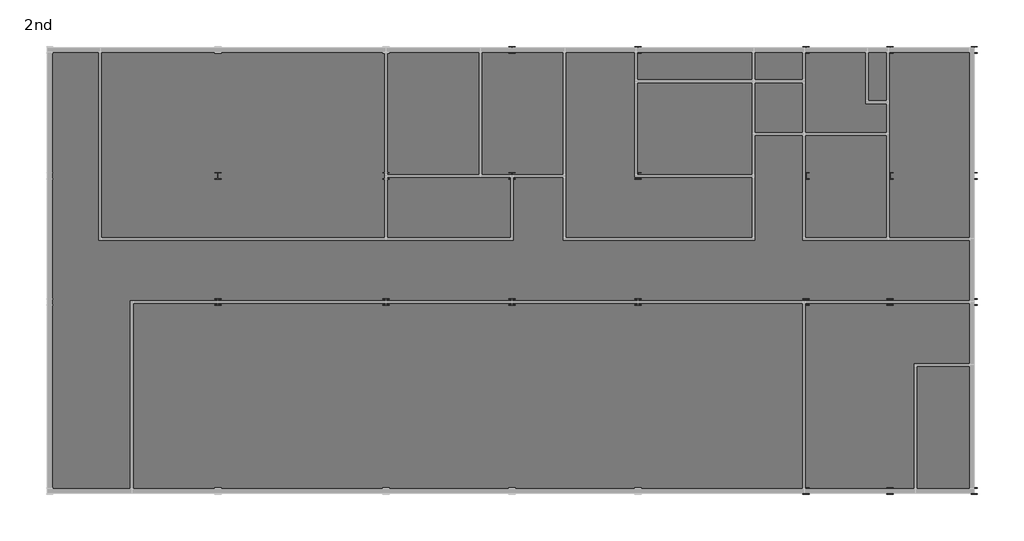
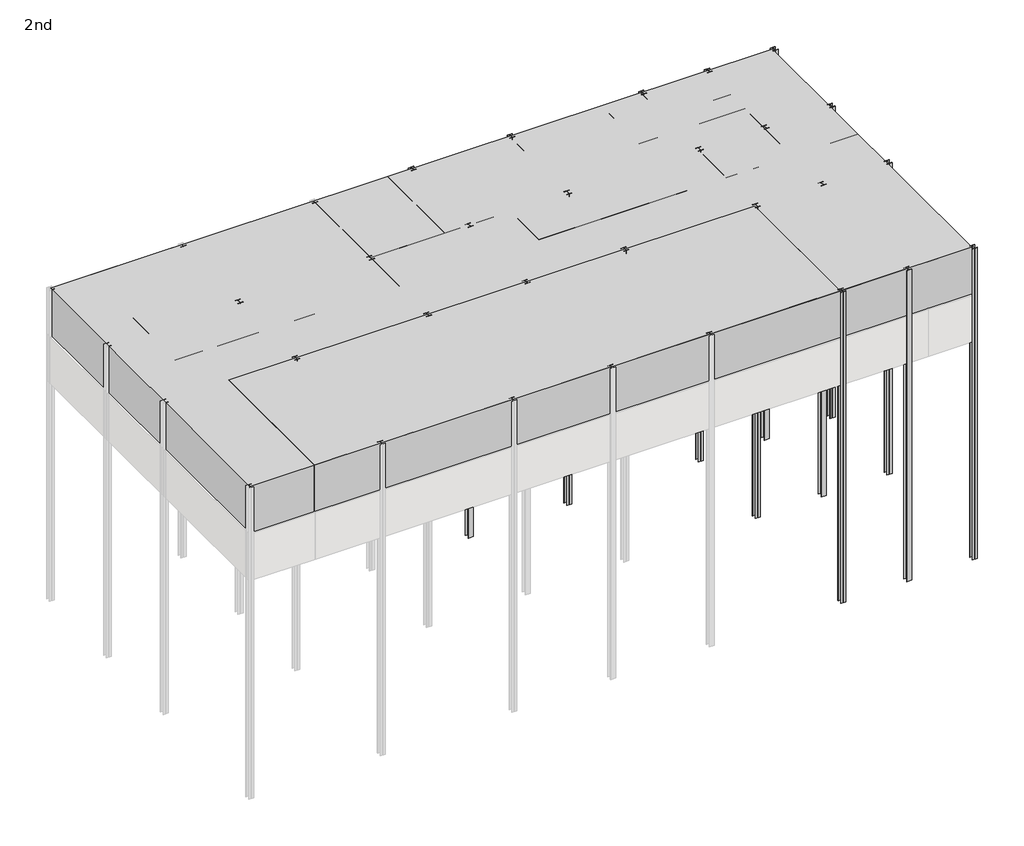
# One storey, part 3 of 3: 17 proxies, 16 columns.
"""IFC4 building model written with IfcOpenShell, lengths in millimetres."""

import ifcopenshell
import ifcopenshell.guid

model = None  # the IFC model being written
_history = None  # IfcOwnerHistory: only IFC2X3 demands one
_inside = {}  # id of a spatial element -> (the spatial element, [elements in it])
_under = {}  # id of a project, library or spatial element -> (it, [spatial elements below it])
_declared = {}  # id of a project -> (the project, [libraries it declares])
_typed = {}  # id of a type object -> (the type object, [elements of that type])
_made_of = {}  # id of a material, layer set ... -> (it, [elements and type objects made of it])


def new_model(schema):
    """Start an empty IFC model of exactly this schema.

    Asked for "IFC4X3", IfcOpenShell would pick the latest addendum, in which some entities
    have other attributes; the version numbers below select the first issue.
    IFC2X3 requires an IfcOwnerHistory on every rooted entity: one is made here for all.
    """
    global model, _history
    if schema == "IFC4X3":
        model = ifcopenshell.file(schema_version=(4, 3, 0, 0))
    else:
        model = ifcopenshell.file(schema=schema)
    _inside.clear()
    _under.clear()
    _declared.clear()
    _typed.clear()
    _made_of.clear()
    _history = None
    if model.schema == "IFC2X3":
        org = make("IfcOrganization", Name="unknown")
        user = make(
            "IfcPersonAndOrganization",
            ThePerson=make("IfcPerson", FamilyName="unknown"),
            TheOrganization=org,
        )
        app = make(
            "IfcApplication",
            ApplicationDeveloper=org,
            Version="unknown",
            ApplicationFullName="unknown",
            ApplicationIdentifier="unknown",
        )
        _history = make(
            "IfcOwnerHistory",
            OwningUser=user,
            OwningApplication=app,
            ChangeAction="ADDED",
            CreationDate=0,
        )
    return model


def make(cls, **values):
    """One entity of the class cls with the attributes given. An attribute that is None is left unset."""
    return model.create_entity(
        cls, **{name: value for name, value in values.items() if value is not None}
    )


def rooted(cls, **values):
    """An entity with a GlobalId (a new one), such as an element, a storey or a relation."""
    return make(cls, GlobalId=ifcopenshell.guid.new(), OwnerHistory=_history, **values)


def si_unit(unit_type, name, prefix=None):
    """IfcSIUnit, for example si_unit("LENGTHUNIT", "METRE", prefix="MILLI")."""
    return make("IfcSIUnit", UnitType=unit_type, Prefix=prefix, Name=name)


def assignment(units):
    """IfcUnitAssignment: the units of a project."""
    return None if units is None else make("IfcUnitAssignment", Units=units)


def point(xyz):
    """IfcCartesianPoint."""
    return None if xyz is None else make("IfcCartesianPoint", Coordinates=xyz)


def direction(xyz):
    """IfcDirection."""
    return None if xyz is None else make("IfcDirection", DirectionRatios=xyz)


def frame(location, z_axis=None, x_axis=None):
    """IfcAxis2Placement3D, a coordinate frame: its origin and axes. An axis left out is left unset."""
    return make(
        "IfcAxis2Placement3D",
        Location=point(location),
        Axis=direction(z_axis),
        RefDirection=direction(x_axis),
    )


def frame_2d(location, x_axis=None):
    """IfcAxis2Placement2D, a coordinate frame in the plane: its origin and x axis."""
    return make(
        "IfcAxis2Placement2D", Location=point(location), RefDirection=direction(x_axis)
    )


def origin():
    """The frame at (0, 0, 0) with its axes left unset."""
    return frame((0.0, 0.0, 0.0))


def origin_with_axes():
    """The frame at (0, 0, 0) with the z axis (0, 0, 1) and the x axis (1, 0, 0) written out."""
    return frame((0.0, 0.0, 0.0), z_axis=(0.0, 0.0, 1.0), x_axis=(1.0, 0.0, 0.0))


def place(relative_to, where):
    """IfcLocalPlacement: puts the frame where relative to a parent placement (None: the world)."""
    return make(
        "IfcLocalPlacement", PlacementRelTo=relative_to, RelativePlacement=where
    )


def context(
    kind, dimensions, precision=None, world=None, true_north=None, identifier=None
):
    """IfcGeometricRepresentationContext, for example the 3D "Model" context."""
    return make(
        "IfcGeometricRepresentationContext",
        ContextIdentifier=identifier,
        ContextType=kind,
        CoordinateSpaceDimension=dimensions,
        Precision=precision,
        WorldCoordinateSystem=world,
        TrueNorth=true_north,
    )


def project(units=None, contexts=None):
    """IfcProject with its units and contexts."""
    return rooted(
        "IfcProject",
        Name="project",
        RepresentationContexts=contexts,
        UnitsInContext=assignment(units),
    )


def spatial(cls, under=None, at=None, **own):
    """A site, building, storey or space (cls), placed at a placement, below another one or the project."""
    s = rooted(cls, ObjectPlacement=at, **own)
    if under is not None:
        _under.setdefault(under.id(), (under, []))[1].append(s)
    return s


def polyline(points):
    """IfcPolyline through the points."""
    return make("IfcPolyline", Points=[point(p) for p in points])


def circle_curve(where, radius):
    """IfcCircle in the frame where."""
    return make("IfcCircle", Position=where, Radius=radius)


def trimmed(basis, trim1, trim2, sense, master):
    """IfcTrimmedCurve: the piece of a basis curve between two trims."""
    return make(
        "IfcTrimmedCurve",
        BasisCurve=basis,
        Trim1=trim1,
        Trim2=trim2,
        SenseAgreement=sense,
        MasterRepresentation=master,
    )


def segment(curve, same_sense, transition):
    """IfcCompositeCurveSegment."""
    return make(
        "IfcCompositeCurveSegment",
        Transition=transition,
        SameSense=same_sense,
        ParentCurve=curve,
    )


def composite_curve(segments, self_intersect=None):
    """IfcCompositeCurve: segments joined end to end."""
    return make("IfcCompositeCurve", Segments=segments, SelfIntersect=self_intersect)


def outline(outer, holes=None, kind="AREA"):
    """IfcArbitraryClosedProfileDef: a profile drawn as a closed curve; with holes, ...WithVoids."""
    if holes is None:
        return make("IfcArbitraryClosedProfileDef", ProfileType=kind, OuterCurve=outer)
    return make(
        "IfcArbitraryProfileDefWithVoids",
        ProfileType=kind,
        OuterCurve=outer,
        InnerCurves=holes,
    )


def extrude(swept, where, along, depth):
    """IfcExtrudedAreaSolid: the profile swept, set in the frame where, extruded along a direction by depth."""
    return make(
        "IfcExtrudedAreaSolid",
        SweptArea=swept,
        Position=where,
        ExtrudedDirection=direction(along),
        Depth=depth,
    )


def shape(context_of_items, identifier, shape_type, items):
    """IfcShapeRepresentation: the items that make up one representation, for example the "Body"."""
    return make(
        "IfcShapeRepresentation",
        ContextOfItems=context_of_items,
        RepresentationIdentifier=identifier,
        RepresentationType=shape_type,
        Items=items,
    )


def source(mapping_origin, context_of_items, identifier, shape_type, items):
    """IfcRepresentationMap: a shape defined once, which mapped items show again and again."""
    return make(
        "IfcRepresentationMap",
        MappingOrigin=mapping_origin,
        MappedRepresentation=shape(context_of_items, identifier, shape_type, items),
    )


def transform(
    local_origin,
    x_axis=None,
    y_axis=None,
    z_axis=None,
    scale=None,
    scale2=None,
    scale3=None,
    uniform=True,
):
    """IfcCartesianTransformationOperator3D, or its non-uniform kind. x_axis, y_axis, z_axis: its Axis1, 2, 3."""
    if uniform:
        return make(
            "IfcCartesianTransformationOperator3D",
            Axis1=direction(x_axis),
            Axis2=direction(y_axis),
            LocalOrigin=point(local_origin),
            Scale=scale,
            Axis3=direction(z_axis),
        )
    return make(
        "IfcCartesianTransformationOperator3DnonUniform",
        Axis1=direction(x_axis),
        Axis2=direction(y_axis),
        LocalOrigin=point(local_origin),
        Scale=scale,
        Axis3=direction(z_axis),
        Scale2=scale2,
        Scale3=scale3,
    )


def mapped(mapping_source, mapping_target):
    """IfcMappedItem: shows the shape of a source again, moved by a transform."""
    return make(
        "IfcMappedItem", MappingSource=mapping_source, MappingTarget=mapping_target
    )


def made_of(thing, what):
    """Note that an element or type object is made of a material, layer set ...; save() writes the relation."""
    if what is not None:
        _made_of.setdefault(what.id(), (what, []))[1].append(thing)
    return thing


def element(
    cls,
    number,
    at=None,
    inside=None,
    cuts=None,
    type_object=None,
    material=None,
    context=None,
    identifier="Body",
    shape_type=None,
    held_by="IfcProductDefinitionShape",
    body=None,
    shapes=None,
    **own,
):
    """One element of the class cls, such as IfcWall. Its Tag is "e" and its number.

    at: its placement. inside: the storey or other place that contains it. cuts: it is an
    opening in that element (IfcRelVoidsElement). A single representation is given by context,
    identifier, shape_type and body (its items); several are given by shapes. held_by: the class
    of the entity that holds the representations. save() writes the other relations.
    """
    e = rooted(cls, Tag="e%d" % number, ObjectPlacement=at, **own)
    if body is not None:
        shapes = [shape(context, identifier, shape_type, body)]
    if shapes is not None:
        e.Representation = make(held_by, Representations=shapes)
    if inside is not None:
        _inside.setdefault(inside.id(), (inside, []))[1].append(e)
    if cuts is not None:
        rooted(
            "IfcRelVoidsElement", RelatingBuildingElement=cuts, RelatedOpeningElement=e
        )
    if type_object is not None:
        _typed.setdefault(type_object.id(), (type_object, []))[1].append(e)
    return made_of(e, material)


def aggregate(whole, parts):
    """IfcRelAggregates: a whole, such as a stair, and the parts it consists of."""
    return rooted("IfcRelAggregates", RelatingObject=whole, RelatedObjects=parts)


def save(model, path):
    """Write the relations noted so far, then the file.

    IfcRelAggregates (storeys below a building ...), IfcRelContainedInSpatialStructure (elements
    in a storey), IfcRelDefinesByType, IfcRelAssociatesMaterial and IfcRelDeclares: one each for
    every whole, place, type object, material and project.
    """
    for whole, parts in _under.values():
        aggregate(whole, parts)
    for where, things in _inside.values():
        rooted(
            "IfcRelContainedInSpatialStructure",
            RelatedElements=things,
            RelatingStructure=where,
        )
    for kind, things in _typed.values():
        rooted("IfcRelDefinesByType", RelatedObjects=things, RelatingType=kind)
    for what, things in _made_of.values():
        rooted("IfcRelAssociatesMaterial", RelatedObjects=things, RelatingMaterial=what)
    for by, libraries in _declared.values():
        rooted("IfcRelDeclares", RelatingContext=by, RelatedDefinitions=libraries)
    model.write(path)


def generic_models_29bcd6f9(model_context):
    return source(origin(), model_context, "Body", "SweptSolid", [
        extrude(outline(polyline([(2000.0, 4500.0), (2000.0, -4500.0), (-2000.0, -4500.0), (-2000.0, 4500.0), (2000.0, 4500.0)])), origin_with_axes(), (0.0, 0.0, 1.0), 6000.0),
    ])


def generic_models_5634f436(model_context):
    return source(origin(), model_context, "Body", "SweptSolid", [
        extrude(outline(polyline([(1350.0, 3000.0), (1350.0, -3000.0), (-1350.0, -3000.0), (-1350.0, 3000.0), (1350.0, 3000.0)])), origin_with_axes(), (0.0, 0.0, 1.0), 6000.0),
    ])


def generic_models_71e2440f(model_context):
    return source(origin(), model_context, "Body", "SweptSolid", [
        extrude(outline(polyline([(500.0, 1250.0), (500.0, -1250.0), (-500.0, -1250.0), (-500.0, 1250.0), (500.0, 1250.0)])), origin_with_axes(), (0.0, 0.0, 1.0), 6000.0),
    ])


def generic_models_57c7875f(model_context):
    return source(origin(), model_context, "Body", "SweptSolid", [
        extrude(outline(polyline([(4500.0, 16000.0), (4500.0, -16000.0), (-4500.0, -16000.0), (-4500.0, 16000.0), (4500.0, 16000.0)])), origin_with_axes(), (0.0, 0.0, 1.0), 6000.0),
    ])


def generic_models_7bff30ad(model_context):
    return source(origin(), model_context, "Body", "SweptSolid", [
        extrude(outline(polyline([(2000.0, 2000.0), (2000.0, -2000.0), (-2000.0, -2000.0), (-2000.0, 2000.0), (2000.0, 2000.0)])), origin_with_axes(), (0.0, 0.0, 1.0), 6000.0),
    ])


def generic_models_5b7b272c(model_context):
    return source(origin(), model_context, "Body", "SweptSolid", [
        extrude(outline(polyline([(2000.0, 2500.0), (2000.0, -2500.0), (-2000.0, -2500.0), (-2000.0, 2500.0), (2000.0, 2500.0)])), origin_with_axes(), (0.0, 0.0, 1.0), 6000.0),
    ])


def generic_models_47b98be1(model_context):
    return source(origin(), model_context, "Body", "SweptSolid", [
        extrude(outline(polyline([(1200.0, 2000.0), (1200.0, -2000.0), (-1200.0, -2000.0), (-1200.0, 2000.0), (1200.0, 2000.0)])), origin_with_axes(), (0.0, 0.0, 1.0), 6000.0),
    ])


def generic_models_7a053eeb(model_context):
    return source(origin(), model_context, "Body", "SweptSolid", [
        extrude(outline(polyline([(1200.0, 750.0), (1200.0, -750.0), (-1200.0, -750.0), (-1200.0, 750.0), (1200.0, 750.0)])), origin_with_axes(), (0.0, 0.0, 1.0), 6000.0),
    ])


def generic_models_ec17d728(model_context):
    return source(origin(), model_context, "Body", "SweptSolid", [
        extrude(outline(polyline([(2800.0, 3000.0), (2800.0, -3000.0), (-2800.0, -3000.0), (-2800.0, 3000.0), (2800.0, 3000.0)])), origin_with_axes(), (0.0, 0.0, 1.0), 6000.0),
    ])


def generic_models_85897e09(model_context):
    return source(origin(), model_context, "Body", "SweptSolid", [
        extrude(outline(polyline([(2800.0, 750.0), (2800.0, -750.0), (-2800.0, -750.0), (-2800.0, 750.0), (2800.0, 750.0)])), origin_with_axes(), (0.0, 0.0, 1.0), 6000.0),
    ])


def generic_models_b79df083(model_context):
    return source(origin(), model_context, "Body", "SweptSolid", [
        extrude(outline(polyline([(4500.0, 4500.0), (4500.0, -4500.0), (-4500.0, -4500.0), (-4500.0, 4500.0), (4500.0, 4500.0)])), origin_with_axes(), (0.0, 0.0, 1.0), 6000.0),
    ])


def generic_models_98b71764(model_context):
    return source(origin(), model_context, "Body", "SweptSolid", [
        extrude(outline(polyline([(2000.0, 3000.0), (2000.0, -3000.0), (-2000.0, -3000.0), (-2000.0, 3000.0), (2000.0, 3000.0)])), origin_with_axes(), (0.0, 0.0, 1.0), 6000.0),
    ])


def generic_models_8af91fed(model_context):
    return source(origin(), model_context, "Body", "SweptSolid", [
        extrude(outline(polyline([(2250.0, 3000.0), (2250.0, -3000.0), (-2250.0, -3000.0), (-2250.0, 3000.0), (2250.0, 3000.0)])), origin_with_axes(), (0.0, 0.0, 1.0), 6000.0),
    ])


def generic_models_542cc789(model_context):
    return source(origin(), model_context, "Body", "SweptSolid", [
        extrude(outline(polyline([(1500.0, 3000.0), (1500.0, -3000.0), (-1500.0, -3000.0), (-1500.0, 3000.0), (1500.0, 3000.0)])), origin_with_axes(), (0.0, 0.0, 1.0), 6000.0),
    ])


def generic_models_af0009da(model_context):
    return source(origin(), model_context, "Body", "SweptSolid", [
        extrude(outline(polyline([(4500.0, 6800.0), (4500.0, -6800.0), (-4500.0, -6800.0), (-4500.0, 6800.0), (4500.0, 6800.0)])), origin_with_axes(), (0.0, 0.0, 1.0), 6000.0),
    ])


def generic_models_4d084078(model_context):
    return source(origin(), model_context, "Body", "SweptSolid", [
        extrude(outline(polyline([(4000.0, 4500.0), (4000.0, -4500.0), (-4000.0, -4500.0), (-4000.0, 4500.0), (4000.0, 4500.0)])), origin_with_axes(), (0.0, 0.0, 1.0), 6000.0),
    ])


def generic_models_b3b0fa1d(model_context):
    return source(origin(), model_context, "Body", "SweptSolid", [
        extrude(outline(polyline([(21950.0, 10500.0), (21950.0, -10500.0), (-21950.0, -10500.0), (-21950.0, 10500.0), (21950.0, 10500.0)])), origin_with_axes(), (0.0, 0.0, 1.0), 6000.0),
    ])


model = new_model("IFC4")

# Units and contexts
model_context = context("Model", 3, world=origin())
ifc_project = project(units=[si_unit("LENGTHUNIT", "METRE", prefix="MILLI")], contexts=[model_context])

# Site, building, storey
site = spatial("IfcSite", under=ifc_project)
building = spatial("IfcBuilding", under=site)
storey = spatial("IfcBuildingStorey", under=building, Name="2nd", Elevation=14000.0)

# Proxies
placement = place(None, origin())
generic_models_shape = generic_models_29bcd6f9(model_context)
element("IfcBuildingElementProxy", 1, Name="Space Planning Box_hec : Space Planning Box_hec", ObjectType="Space Planning Box_hec : Space Planning Box_hec", at=placement, inside=storey, context=model_context, shape_type="MappedRepresentation", body=[
    mapped(generic_models_shape, transform((198014.1020501, 147515.7581198, 14000.0), x_axis=(1.0, 0.0, 0.0), y_axis=(0.0, 1.0, 0.0), z_axis=(0.0, 0.0, 1.0))),
])
generic_models_2_shape = generic_models_5634f436(model_context)
element("IfcBuildingElementProxy", 2, Name="Space Planning Box_hec : Space Planning Box_hec", ObjectType="Space Planning Box_hec : Space Planning Box_hec", at=placement, inside=storey, context=model_context, shape_type="MappedRepresentation", body=[
    mapped(generic_models_2_shape, transform((198664.1020501, 134015.7581198, 14000.0), x_axis=(1.0, 0.0, 0.0), y_axis=(0.0, 1.0, 0.0), z_axis=(0.0, 0.0, 1.0))),
])
generic_models_3_shape = generic_models_71e2440f(model_context)
element("IfcBuildingElementProxy", 3, Name="Space Planning Box_hec : Space Planning Box_hec", ObjectType="Space Planning Box_hec : Space Planning Box_hec", at=placement, inside=storey, context=model_context, shape_type="MappedRepresentation", body=[
    mapped(generic_models_3_shape, transform((195514.1020501, 150765.7581198, 14000.0), x_axis=(1.0, 0.0, 0.0), y_axis=(0.0, 1.0, 0.0), z_axis=(0.0, 0.0, 1.0))),
])
generic_models_4_shape = generic_models_57c7875f(model_context)
element("IfcBuildingElementProxy", 4, Name="Space Planning Box_hec : Space Planning Box_hec", ObjectType="Space Planning Box_hec : Space Planning Box_hec", at=placement, inside=storey, context=model_context, shape_type="MappedRepresentation", body=[
    mapped(generic_models_4_shape, transform((176014.1020501, 135515.7581198, 14000.0), x_axis=(0.0, -1.0, 0.0), y_axis=(1.0, 0.0, 0.0), z_axis=(0.0, 0.0, 1.0))),
])
generic_models_5_shape = generic_models_7bff30ad(model_context)
element("IfcBuildingElementProxy", 5, Name="Space Planning Box_hec : Space Planning Box_hec", ObjectType="Space Planning Box_hec : Space Planning Box_hec", at=placement, inside=storey, context=model_context, shape_type="MappedRepresentation", body=[
    mapped(generic_models_5_shape, transform((194014.1020501, 150015.7581198, 14000.0), x_axis=(1.0, 0.0, 0.0), y_axis=(0.0, 1.0, 0.0), z_axis=(0.0, 0.0, 1.0))),
])
generic_models_6_shape = generic_models_5b7b272c(model_context)
element("IfcBuildingElementProxy", 6, Name="Space Planning Box_hec : Space Planning Box_hec", ObjectType="Space Planning Box_hec : Space Planning Box_hec", at=placement, inside=storey, context=model_context, shape_type="MappedRepresentation", body=[
    mapped(generic_models_6_shape, transform((194014.1020501, 145515.7581198, 14000.0), x_axis=(1.0, 0.0, 0.0), y_axis=(0.0, 1.0, 0.0), z_axis=(0.0, 0.0, 1.0))),
])
generic_models_7_shape = generic_models_47b98be1(model_context)
element("IfcBuildingElementProxy", 7, Name="Space Planning Box_hec : Space Planning Box_hec", ObjectType="Space Planning Box_hec : Space Planning Box_hec", at=placement, inside=storey, context=model_context, shape_type="MappedRepresentation", body=[
    mapped(generic_models_7_shape, transform((190814.1020501, 150015.7581198, 14000.0), x_axis=(1.0, 0.0, 0.0), y_axis=(0.0, 1.0, 0.0), z_axis=(0.0, 0.0, 1.0))),
])
generic_models_8_shape = generic_models_7a053eeb(model_context)
element("IfcBuildingElementProxy", 8, Name="Space Planning Box_hec : Space Planning Box_hec", ObjectType="Space Planning Box_hec : Space Planning Box_hec", at=placement, inside=storey, context=model_context, shape_type="MappedRepresentation", body=[
    mapped(generic_models_8_shape, transform((190814.1020501, 151265.7581198, 14000.0), x_axis=(1.0, 0.0, 0.0), y_axis=(0.0, 1.0, 0.0), z_axis=(0.0, 0.0, 1.0))),
])
generic_models_9_shape = generic_models_ec17d728(model_context)
element("IfcBuildingElementProxy", 9, Name="Space Planning Box_hec : Space Planning Box_hec", ObjectType="Space Planning Box_hec : Space Planning Box_hec", at=placement, inside=storey, context=model_context, shape_type="MappedRepresentation", body=[
    mapped(generic_models_9_shape, transform((186814.1020501, 149015.7581198, 14000.0), x_axis=(1.0, 0.0, 0.0), y_axis=(0.0, 1.0, 0.0), z_axis=(0.0, 0.0, 1.0))),
])
generic_models_10_shape = generic_models_85897e09(model_context)
element("IfcBuildingElementProxy", 10, Name="Space Planning Box_hec : Space Planning Box_hec", ObjectType="Space Planning Box_hec : Space Planning Box_hec", at=placement, inside=storey, context=model_context, shape_type="MappedRepresentation", body=[
    mapped(generic_models_10_shape, transform((186814.1020501, 151265.7581198, 14000.0), x_axis=(1.0, 0.0, 0.0), y_axis=(0.0, 1.0, 0.0), z_axis=(0.0, 0.0, 1.0))),
])
generic_models_11_shape = generic_models_b79df083(model_context)
element("IfcBuildingElementProxy", 11, Name="Space Planning Box_hec : Space Planning Box_hec", ObjectType="Space Planning Box_hec : Space Planning Box_hec", at=placement, inside=storey, context=model_context, shape_type="MappedRepresentation", body=[
    mapped(generic_models_11_shape, transform((185114.1020501, 147515.7581198, 14000.0), x_axis=(1.0, 0.0, 0.0), y_axis=(0.0, 1.0, 0.0), z_axis=(0.0, 0.0, 1.0))),
])
generic_models_12_shape = generic_models_98b71764(model_context)
element("IfcBuildingElementProxy", 12, Name="Space Planning Box_hec : Space Planning Box_hec", ObjectType="Space Planning Box_hec : Space Planning Box_hec", at=placement, inside=storey, context=model_context, shape_type="MappedRepresentation", body=[
    mapped(generic_models_12_shape, transform((178614.1020501, 149015.7581198, 14000.0), x_axis=(1.0, 0.0, 0.0), y_axis=(0.0, 1.0, 0.0), z_axis=(0.0, 0.0, 1.0))),
])
generic_models_13_shape = generic_models_8af91fed(model_context)
element("IfcBuildingElementProxy", 13, Name="Space Planning Box_hec : Space Planning Box_hec", ObjectType="Space Planning Box_hec : Space Planning Box_hec", at=placement, inside=storey, context=model_context, shape_type="MappedRepresentation", body=[
    mapped(generic_models_13_shape, transform((174364.1020501, 149015.7581198, 14000.0), x_axis=(1.0, 0.0, 0.0), y_axis=(0.0, 1.0, 0.0), z_axis=(0.0, 0.0, 1.0))),
])
generic_models_14_shape = generic_models_542cc789(model_context)
element("IfcBuildingElementProxy", 14, Name="Space Planning Box_hec : Space Planning Box_hec", ObjectType="Space Planning Box_hec : Space Planning Box_hec", at=placement, inside=storey, context=model_context, shape_type="MappedRepresentation", body=[
    mapped(generic_models_14_shape, transform((175114.1020501, 144515.7581198, 14000.0), x_axis=(0.0, 1.0, 0.0), y_axis=(-1.0, 0.0, 0.0), z_axis=(0.0, 0.0, 1.0))),
])
generic_models_15_shape = generic_models_af0009da(model_context)
element("IfcBuildingElementProxy", 15, Name="Space Planning Box_hec : Space Planning Box_hec", ObjectType="Space Planning Box_hec : Space Planning Box_hec", at=placement, inside=storey, context=model_context, shape_type="MappedRepresentation", body=[
    mapped(generic_models_15_shape, transform((165314.1020501, 147515.7581198, 14000.0), x_axis=(0.0, -1.0, 0.0), y_axis=(1.0, 0.0, 0.0), z_axis=(0.0, 0.0, 1.0))),
])
generic_models_16_shape = generic_models_4d084078(model_context)
element("IfcBuildingElementProxy", 16, Name="Space Planning Box_hec : Space Planning Box_hec", ObjectType="Space Planning Box_hec : Space Planning Box_hec", at=placement, inside=storey, context=model_context, shape_type="MappedRepresentation", body=[
    mapped(generic_models_16_shape, transform((196014.1020501, 135515.7581198, 14000.0), x_axis=(1.0, 0.0, 0.0), y_axis=(0.0, 1.0, 0.0), z_axis=(0.0, 0.0, 1.0))),
])
generic_models_17_shape = generic_models_b3b0fa1d(model_context)
element("IfcBuildingElementProxy", 17, Name="Space Planning Box_hec : Space Planning Box_hec", ObjectType="Space Planning Box_hec : Space Planning Box_hec", at=placement, inside=storey, context=model_context, shape_type="MappedRepresentation", body=[
    mapped(generic_models_17_shape, transform((178064.1020501, 141515.7581198, 14000.0), x_axis=(1.0, 0.0, 0.0), y_axis=(0.0, 1.0, 0.0), z_axis=(0.0, 0.0, 1.0))),
])

# Columns
element("IfcColumn", 18, ObjectType="UC-Universal Columns-Column : UC305x305x97", at=placement, inside=storey, context=model_context, shape_type="SweptSolid", body=[
    extrude(outline(composite_curve([segment(polyline([(178266.7520501, 152169.7081198), (178266.7520501, 152154.3081198), (178134.2520501, 152154.3081198)]), True, "CONTINUOUS"), segment(trimmed(circle_curve(frame_2d((178134.2520501, 152139.1081198)), 15.2), [point((178134.2520501, 152154.3081198))], [point((178119.0520501, 152139.1081198))], True, "CARTESIAN"), True, "CONTINUOUS"), segment(polyline([(178119.0520501, 152139.1081198), (178119.0520501, 151892.4081198)]), True, "CONTINUOUS"), segment(trimmed(circle_curve(frame_2d((178134.2520501, 151892.4081198)), 15.2), [point((178119.0520501, 151892.4081198))], [point((178134.2520501, 151877.2081198))], True, "CARTESIAN"), True, "CONTINUOUS"), segment(polyline([(178134.2520501, 151877.2081198), (178266.7520501, 151877.2081198), (178266.7520501, 151861.8081198), (177961.4520501, 151861.8081198), (177961.4520501, 151877.2081198), (178093.9520501, 151877.2081198)]), True, "CONTINUOUS"), segment(trimmed(circle_curve(frame_2d((178093.9520501, 151892.4081198)), 15.2), [point((178093.9520501, 151877.2081198))], [point((178109.1520501, 151892.4081198))], True, "CARTESIAN"), True, "CONTINUOUS"), segment(polyline([(178109.1520501, 151892.4081198), (178109.1520501, 152139.1081198)]), True, "CONTINUOUS"), segment(trimmed(circle_curve(frame_2d((178093.9520501, 152139.1081198)), 15.2), [point((178109.1520501, 152139.1081198))], [point((178093.9520501, 152154.3081198))], True, "CARTESIAN"), True, "CONTINUOUS"), segment(polyline([(178093.9520501, 152154.3081198), (177961.4520501, 152154.3081198), (177961.4520501, 152169.7081198), (178266.7520501, 152169.7081198)]), True, "CONTINUOUS")], self_intersect=False)), origin_with_axes(), (0.0, 0.0, 1.0), 20000.0),
])
element("IfcColumn", 19, ObjectType="UC-Universal Columns-Column : UC305x305x97", at=placement, inside=storey, context=model_context, shape_type="SweptSolid", body=[
    extrude(outline(composite_curve([segment(polyline([(178266.7520501, 146169.7081198), (178266.7520501, 146154.3081198), (178134.2520501, 146154.3081198)]), True, "CONTINUOUS"), segment(trimmed(circle_curve(frame_2d((178134.2520501, 146139.1081198)), 15.2), [point((178134.2520501, 146154.3081198))], [point((178119.0520501, 146139.1081198))], True, "CARTESIAN"), True, "CONTINUOUS"), segment(polyline([(178119.0520501, 146139.1081198), (178119.0520501, 145892.4081198)]), True, "CONTINUOUS"), segment(trimmed(circle_curve(frame_2d((178134.2520501, 145892.4081198)), 15.2), [point((178119.0520501, 145892.4081198))], [point((178134.2520501, 145877.2081198))], True, "CARTESIAN"), True, "CONTINUOUS"), segment(polyline([(178134.2520501, 145877.2081198), (178266.7520501, 145877.2081198), (178266.7520501, 145861.8081198), (177961.4520501, 145861.8081198), (177961.4520501, 145877.2081198), (178093.9520501, 145877.2081198)]), True, "CONTINUOUS"), segment(trimmed(circle_curve(frame_2d((178093.9520501, 145892.4081198)), 15.2), [point((178093.9520501, 145877.2081198))], [point((178109.1520501, 145892.4081198))], True, "CARTESIAN"), True, "CONTINUOUS"), segment(polyline([(178109.1520501, 145892.4081198), (178109.1520501, 146139.1081198)]), True, "CONTINUOUS"), segment(trimmed(circle_curve(frame_2d((178093.9520501, 146139.1081198)), 15.2), [point((178109.1520501, 146139.1081198))], [point((178093.9520501, 146154.3081198))], True, "CARTESIAN"), True, "CONTINUOUS"), segment(polyline([(178093.9520501, 146154.3081198), (177961.4520501, 146154.3081198), (177961.4520501, 146169.7081198), (178266.7520501, 146169.7081198)]), True, "CONTINUOUS")], self_intersect=False)), origin_with_axes(), (0.0, 0.0, 1.0), 20000.0),
])
element("IfcColumn", 20, ObjectType="UC-Universal Columns-Column : UC305x305x97", at=placement, inside=storey, context=model_context, shape_type="SweptSolid", body=[
    extrude(outline(composite_curve([segment(polyline([(184266.7520501, 152169.7081198), (184266.7520501, 152154.3081198), (184134.2520501, 152154.3081198)]), True, "CONTINUOUS"), segment(trimmed(circle_curve(frame_2d((184134.2520501, 152139.1081198)), 15.2), [point((184134.2520501, 152154.3081198))], [point((184119.0520501, 152139.1081198))], True, "CARTESIAN"), True, "CONTINUOUS"), segment(polyline([(184119.0520501, 152139.1081198), (184119.0520501, 151892.4081198)]), True, "CONTINUOUS"), segment(trimmed(circle_curve(frame_2d((184134.2520501, 151892.4081198)), 15.2), [point((184119.0520501, 151892.4081198))], [point((184134.2520501, 151877.2081198))], True, "CARTESIAN"), True, "CONTINUOUS"), segment(polyline([(184134.2520501, 151877.2081198), (184266.7520501, 151877.2081198), (184266.7520501, 151861.8081198), (183961.4520501, 151861.8081198), (183961.4520501, 151877.2081198), (184093.9520501, 151877.2081198)]), True, "CONTINUOUS"), segment(trimmed(circle_curve(frame_2d((184093.9520501, 151892.4081198)), 15.2), [point((184093.9520501, 151877.2081198))], [point((184109.1520501, 151892.4081198))], True, "CARTESIAN"), True, "CONTINUOUS"), segment(polyline([(184109.1520501, 151892.4081198), (184109.1520501, 152139.1081198)]), True, "CONTINUOUS"), segment(trimmed(circle_curve(frame_2d((184093.9520501, 152139.1081198)), 15.2), [point((184109.1520501, 152139.1081198))], [point((184093.9520501, 152154.3081198))], True, "CARTESIAN"), True, "CONTINUOUS"), segment(polyline([(184093.9520501, 152154.3081198), (183961.4520501, 152154.3081198), (183961.4520501, 152169.7081198), (184266.7520501, 152169.7081198)]), True, "CONTINUOUS")], self_intersect=False)), origin_with_axes(), (0.0, 0.0, 1.0), 20000.0),
])
element("IfcColumn", 21, ObjectType="UC-Universal Columns-Column : UC305x305x97", at=placement, inside=storey, context=model_context, shape_type="SweptSolid", body=[
    extrude(outline(composite_curve([segment(polyline([(184266.7520501, 146169.7081198), (184266.7520501, 146154.3081198), (184134.2520501, 146154.3081198)]), True, "CONTINUOUS"), segment(trimmed(circle_curve(frame_2d((184134.2520501, 146139.1081198)), 15.2), [point((184134.2520501, 146154.3081198))], [point((184119.0520501, 146139.1081198))], True, "CARTESIAN"), True, "CONTINUOUS"), segment(polyline([(184119.0520501, 146139.1081198), (184119.0520501, 145892.4081198)]), True, "CONTINUOUS"), segment(trimmed(circle_curve(frame_2d((184134.2520501, 145892.4081198)), 15.2), [point((184119.0520501, 145892.4081198))], [point((184134.2520501, 145877.2081198))], True, "CARTESIAN"), True, "CONTINUOUS"), segment(polyline([(184134.2520501, 145877.2081198), (184266.7520501, 145877.2081198), (184266.7520501, 145861.8081198), (183961.4520501, 145861.8081198), (183961.4520501, 145877.2081198), (184093.9520501, 145877.2081198)]), True, "CONTINUOUS"), segment(trimmed(circle_curve(frame_2d((184093.9520501, 145892.4081198)), 15.2), [point((184093.9520501, 145877.2081198))], [point((184109.1520501, 145892.4081198))], True, "CARTESIAN"), True, "CONTINUOUS"), segment(polyline([(184109.1520501, 145892.4081198), (184109.1520501, 146139.1081198)]), True, "CONTINUOUS"), segment(trimmed(circle_curve(frame_2d((184093.9520501, 146139.1081198)), 15.2), [point((184109.1520501, 146139.1081198))], [point((184093.9520501, 146154.3081198))], True, "CARTESIAN"), True, "CONTINUOUS"), segment(polyline([(184093.9520501, 146154.3081198), (183961.4520501, 146154.3081198), (183961.4520501, 146169.7081198), (184266.7520501, 146169.7081198)]), True, "CONTINUOUS")], self_intersect=False)), origin_with_axes(), (0.0, 0.0, 1.0), 20000.0),
])
element("IfcColumn", 22, ObjectType="UC-Universal Columns-Column : UC305x305x97", at=placement, inside=storey, context=model_context, shape_type="SweptSolid", body=[
    extrude(outline(composite_curve([segment(polyline([(192266.7520501, 152169.7081198), (192266.7520501, 152154.3081198), (192134.2520501, 152154.3081198)]), True, "CONTINUOUS"), segment(trimmed(circle_curve(frame_2d((192134.2520501, 152139.1081198)), 15.2), [point((192134.2520501, 152154.3081198))], [point((192119.0520501, 152139.1081198))], True, "CARTESIAN"), True, "CONTINUOUS"), segment(polyline([(192119.0520501, 152139.1081198), (192119.0520501, 151892.4081198)]), True, "CONTINUOUS"), segment(trimmed(circle_curve(frame_2d((192134.2520501, 151892.4081198)), 15.2), [point((192119.0520501, 151892.4081198))], [point((192134.2520501, 151877.2081198))], True, "CARTESIAN"), True, "CONTINUOUS"), segment(polyline([(192134.2520501, 151877.2081198), (192266.7520501, 151877.2081198), (192266.7520501, 151861.8081198), (191961.4520501, 151861.8081198), (191961.4520501, 151877.2081198), (192093.9520501, 151877.2081198)]), True, "CONTINUOUS"), segment(trimmed(circle_curve(frame_2d((192093.9520501, 151892.4081198)), 15.2), [point((192093.9520501, 151877.2081198))], [point((192109.1520501, 151892.4081198))], True, "CARTESIAN"), True, "CONTINUOUS"), segment(polyline([(192109.1520501, 151892.4081198), (192109.1520501, 152139.1081198)]), True, "CONTINUOUS"), segment(trimmed(circle_curve(frame_2d((192093.9520501, 152139.1081198)), 15.2), [point((192109.1520501, 152139.1081198))], [point((192093.9520501, 152154.3081198))], True, "CARTESIAN"), True, "CONTINUOUS"), segment(polyline([(192093.9520501, 152154.3081198), (191961.4520501, 152154.3081198), (191961.4520501, 152169.7081198), (192266.7520501, 152169.7081198)]), True, "CONTINUOUS")], self_intersect=False)), origin_with_axes(), (0.0, 0.0, 1.0), 20000.0),
])
element("IfcColumn", 23, ObjectType="UC-Universal Columns-Column : UC305x305x97", at=placement, inside=storey, context=model_context, shape_type="SweptSolid", body=[
    extrude(outline(composite_curve([segment(polyline([(192266.7520501, 146169.7081198), (192266.7520501, 146154.3081198), (192134.2520501, 146154.3081198)]), True, "CONTINUOUS"), segment(trimmed(circle_curve(frame_2d((192134.2520501, 146139.1081198)), 15.2), [point((192134.2520501, 146154.3081198))], [point((192119.0520501, 146139.1081198))], True, "CARTESIAN"), True, "CONTINUOUS"), segment(polyline([(192119.0520501, 146139.1081198), (192119.0520501, 145892.4081198)]), True, "CONTINUOUS"), segment(trimmed(circle_curve(frame_2d((192134.2520501, 145892.4081198)), 15.2), [point((192119.0520501, 145892.4081198))], [point((192134.2520501, 145877.2081198))], True, "CARTESIAN"), True, "CONTINUOUS"), segment(polyline([(192134.2520501, 145877.2081198), (192266.7520501, 145877.2081198), (192266.7520501, 145861.8081198), (191961.4520501, 145861.8081198), (191961.4520501, 145877.2081198), (192093.9520501, 145877.2081198)]), True, "CONTINUOUS"), segment(trimmed(circle_curve(frame_2d((192093.9520501, 145892.4081198)), 15.2), [point((192093.9520501, 145877.2081198))], [point((192109.1520501, 145892.4081198))], True, "CARTESIAN"), True, "CONTINUOUS"), segment(polyline([(192109.1520501, 145892.4081198), (192109.1520501, 146139.1081198)]), True, "CONTINUOUS"), segment(trimmed(circle_curve(frame_2d((192093.9520501, 146139.1081198)), 15.2), [point((192109.1520501, 146139.1081198))], [point((192093.9520501, 146154.3081198))], True, "CARTESIAN"), True, "CONTINUOUS"), segment(polyline([(192093.9520501, 146154.3081198), (191961.4520501, 146154.3081198), (191961.4520501, 146169.7081198), (192266.7520501, 146169.7081198)]), True, "CONTINUOUS")], self_intersect=False)), origin_with_axes(), (0.0, 0.0, 1.0), 20000.0),
])
element("IfcColumn", 24, ObjectType="UC-Universal Columns-Column : UC305x305x97", at=placement, inside=storey, context=model_context, shape_type="SweptSolid", body=[
    extrude(outline(composite_curve([segment(polyline([(192266.7520501, 140169.7081198), (192266.7520501, 140154.3081198), (192134.2520501, 140154.3081198)]), True, "CONTINUOUS"), segment(trimmed(circle_curve(frame_2d((192134.2520501, 140139.1081198)), 15.2), [point((192134.2520501, 140154.3081198))], [point((192119.0520501, 140139.1081198))], True, "CARTESIAN"), True, "CONTINUOUS"), segment(polyline([(192119.0520501, 140139.1081198), (192119.0520501, 139892.4081198)]), True, "CONTINUOUS"), segment(trimmed(circle_curve(frame_2d((192134.2520501, 139892.4081198)), 15.2), [point((192119.0520501, 139892.4081198))], [point((192134.2520501, 139877.2081198))], True, "CARTESIAN"), True, "CONTINUOUS"), segment(polyline([(192134.2520501, 139877.2081198), (192266.7520501, 139877.2081198), (192266.7520501, 139861.8081198), (191961.4520501, 139861.8081198), (191961.4520501, 139877.2081198), (192093.9520501, 139877.2081198)]), True, "CONTINUOUS"), segment(trimmed(circle_curve(frame_2d((192093.9520501, 139892.4081198)), 15.2), [point((192093.9520501, 139877.2081198))], [point((192109.1520501, 139892.4081198))], True, "CARTESIAN"), True, "CONTINUOUS"), segment(polyline([(192109.1520501, 139892.4081198), (192109.1520501, 140139.1081198)]), True, "CONTINUOUS"), segment(trimmed(circle_curve(frame_2d((192093.9520501, 140139.1081198)), 15.2), [point((192109.1520501, 140139.1081198))], [point((192093.9520501, 140154.3081198))], True, "CARTESIAN"), True, "CONTINUOUS"), segment(polyline([(192093.9520501, 140154.3081198), (191961.4520501, 140154.3081198), (191961.4520501, 140169.7081198), (192266.7520501, 140169.7081198)]), True, "CONTINUOUS")], self_intersect=False)), origin_with_axes(), (0.0, 0.0, 1.0), 20000.0),
])
element("IfcColumn", 25, ObjectType="UC-Universal Columns-Column : UC305x305x97", at=placement, inside=storey, context=model_context, shape_type="SweptSolid", body=[
    extrude(outline(composite_curve([segment(polyline([(192266.7520501, 131169.7081198), (192266.7520501, 131154.3081198), (192134.2520501, 131154.3081198)]), True, "CONTINUOUS"), segment(trimmed(circle_curve(frame_2d((192134.2520501, 131139.1081198)), 15.2), [point((192134.2520501, 131154.3081198))], [point((192119.0520501, 131139.1081198))], True, "CARTESIAN"), True, "CONTINUOUS"), segment(polyline([(192119.0520501, 131139.1081198), (192119.0520501, 130892.4081198)]), True, "CONTINUOUS"), segment(trimmed(circle_curve(frame_2d((192134.2520501, 130892.4081198)), 15.2), [point((192119.0520501, 130892.4081198))], [point((192134.2520501, 130877.2081198))], True, "CARTESIAN"), True, "CONTINUOUS"), segment(polyline([(192134.2520501, 130877.2081198), (192266.7520501, 130877.2081198), (192266.7520501, 130861.8081198), (191961.4520501, 130861.8081198), (191961.4520501, 130877.2081198), (192093.9520501, 130877.2081198)]), True, "CONTINUOUS"), segment(trimmed(circle_curve(frame_2d((192093.9520501, 130892.4081198)), 15.2), [point((192093.9520501, 130877.2081198))], [point((192109.1520501, 130892.4081198))], True, "CARTESIAN"), True, "CONTINUOUS"), segment(polyline([(192109.1520501, 130892.4081198), (192109.1520501, 131139.1081198)]), True, "CONTINUOUS"), segment(trimmed(circle_curve(frame_2d((192093.9520501, 131139.1081198)), 15.2), [point((192109.1520501, 131139.1081198))], [point((192093.9520501, 131154.3081198))], True, "CARTESIAN"), True, "CONTINUOUS"), segment(polyline([(192093.9520501, 131154.3081198), (191961.4520501, 131154.3081198), (191961.4520501, 131169.7081198), (192266.7520501, 131169.7081198)]), True, "CONTINUOUS")], self_intersect=False)), origin_with_axes(), (0.0, 0.0, 1.0), 20000.0),
])
element("IfcColumn", 26, ObjectType="UC-Universal Columns-Column : UC305x305x97", at=placement, inside=storey, context=model_context, shape_type="SweptSolid", body=[
    extrude(outline(composite_curve([segment(polyline([(196266.7520501, 152169.7081198), (196266.7520501, 152154.3081198), (196134.2520501, 152154.3081198)]), True, "CONTINUOUS"), segment(trimmed(circle_curve(frame_2d((196134.2520501, 152139.1081198)), 15.2), [point((196134.2520501, 152154.3081198))], [point((196119.0520501, 152139.1081198))], True, "CARTESIAN"), True, "CONTINUOUS"), segment(polyline([(196119.0520501, 152139.1081198), (196119.0520501, 151892.4081198)]), True, "CONTINUOUS"), segment(trimmed(circle_curve(frame_2d((196134.2520501, 151892.4081198)), 15.2), [point((196119.0520501, 151892.4081198))], [point((196134.2520501, 151877.2081198))], True, "CARTESIAN"), True, "CONTINUOUS"), segment(polyline([(196134.2520501, 151877.2081198), (196266.7520501, 151877.2081198), (196266.7520501, 151861.8081198), (195961.4520501, 151861.8081198), (195961.4520501, 151877.2081198), (196093.9520501, 151877.2081198)]), True, "CONTINUOUS"), segment(trimmed(circle_curve(frame_2d((196093.9520501, 151892.4081198)), 15.2), [point((196093.9520501, 151877.2081198))], [point((196109.1520501, 151892.4081198))], True, "CARTESIAN"), True, "CONTINUOUS"), segment(polyline([(196109.1520501, 151892.4081198), (196109.1520501, 152139.1081198)]), True, "CONTINUOUS"), segment(trimmed(circle_curve(frame_2d((196093.9520501, 152139.1081198)), 15.2), [point((196109.1520501, 152139.1081198))], [point((196093.9520501, 152154.3081198))], True, "CARTESIAN"), True, "CONTINUOUS"), segment(polyline([(196093.9520501, 152154.3081198), (195961.4520501, 152154.3081198), (195961.4520501, 152169.7081198), (196266.7520501, 152169.7081198)]), True, "CONTINUOUS")], self_intersect=False)), origin_with_axes(), (0.0, 0.0, 1.0), 20000.0),
])
element("IfcColumn", 27, ObjectType="UC-Universal Columns-Column : UC305x305x97", at=placement, inside=storey, context=model_context, shape_type="SweptSolid", body=[
    extrude(outline(composite_curve([segment(polyline([(196266.7520501, 146169.7081198), (196266.7520501, 146154.3081198), (196134.2520501, 146154.3081198)]), True, "CONTINUOUS"), segment(trimmed(circle_curve(frame_2d((196134.2520501, 146139.1081198)), 15.2), [point((196134.2520501, 146154.3081198))], [point((196119.0520501, 146139.1081198))], True, "CARTESIAN"), True, "CONTINUOUS"), segment(polyline([(196119.0520501, 146139.1081198), (196119.0520501, 145892.4081198)]), True, "CONTINUOUS"), segment(trimmed(circle_curve(frame_2d((196134.2520501, 145892.4081198)), 15.2), [point((196119.0520501, 145892.4081198))], [point((196134.2520501, 145877.2081198))], True, "CARTESIAN"), True, "CONTINUOUS"), segment(polyline([(196134.2520501, 145877.2081198), (196266.7520501, 145877.2081198), (196266.7520501, 145861.8081198), (195961.4520501, 145861.8081198), (195961.4520501, 145877.2081198), (196093.9520501, 145877.2081198)]), True, "CONTINUOUS"), segment(trimmed(circle_curve(frame_2d((196093.9520501, 145892.4081198)), 15.2), [point((196093.9520501, 145877.2081198))], [point((196109.1520501, 145892.4081198))], True, "CARTESIAN"), True, "CONTINUOUS"), segment(polyline([(196109.1520501, 145892.4081198), (196109.1520501, 146139.1081198)]), True, "CONTINUOUS"), segment(trimmed(circle_curve(frame_2d((196093.9520501, 146139.1081198)), 15.2), [point((196109.1520501, 146139.1081198))], [point((196093.9520501, 146154.3081198))], True, "CARTESIAN"), True, "CONTINUOUS"), segment(polyline([(196093.9520501, 146154.3081198), (195961.4520501, 146154.3081198), (195961.4520501, 146169.7081198), (196266.7520501, 146169.7081198)]), True, "CONTINUOUS")], self_intersect=False)), origin_with_axes(), (0.0, 0.0, 1.0), 20000.0),
])
element("IfcColumn", 28, ObjectType="UC-Universal Columns-Column : UC305x305x97", at=placement, inside=storey, context=model_context, shape_type="SweptSolid", body=[
    extrude(outline(composite_curve([segment(polyline([(196266.7520501, 140169.7081198), (196266.7520501, 140154.3081198), (196134.2520501, 140154.3081198)]), True, "CONTINUOUS"), segment(trimmed(circle_curve(frame_2d((196134.2520501, 140139.1081198)), 15.2), [point((196134.2520501, 140154.3081198))], [point((196119.0520501, 140139.1081198))], True, "CARTESIAN"), True, "CONTINUOUS"), segment(polyline([(196119.0520501, 140139.1081198), (196119.0520501, 139892.4081198)]), True, "CONTINUOUS"), segment(trimmed(circle_curve(frame_2d((196134.2520501, 139892.4081198)), 15.2), [point((196119.0520501, 139892.4081198))], [point((196134.2520501, 139877.2081198))], True, "CARTESIAN"), True, "CONTINUOUS"), segment(polyline([(196134.2520501, 139877.2081198), (196266.7520501, 139877.2081198), (196266.7520501, 139861.8081198), (195961.4520501, 139861.8081198), (195961.4520501, 139877.2081198), (196093.9520501, 139877.2081198)]), True, "CONTINUOUS"), segment(trimmed(circle_curve(frame_2d((196093.9520501, 139892.4081198)), 15.2), [point((196093.9520501, 139877.2081198))], [point((196109.1520501, 139892.4081198))], True, "CARTESIAN"), True, "CONTINUOUS"), segment(polyline([(196109.1520501, 139892.4081198), (196109.1520501, 140139.1081198)]), True, "CONTINUOUS"), segment(trimmed(circle_curve(frame_2d((196093.9520501, 140139.1081198)), 15.2), [point((196109.1520501, 140139.1081198))], [point((196093.9520501, 140154.3081198))], True, "CARTESIAN"), True, "CONTINUOUS"), segment(polyline([(196093.9520501, 140154.3081198), (195961.4520501, 140154.3081198), (195961.4520501, 140169.7081198), (196266.7520501, 140169.7081198)]), True, "CONTINUOUS")], self_intersect=False)), origin_with_axes(), (0.0, 0.0, 1.0), 20000.0),
])
element("IfcColumn", 29, ObjectType="UC-Universal Columns-Column : UC305x305x97", at=placement, inside=storey, context=model_context, shape_type="SweptSolid", body=[
    extrude(outline(composite_curve([segment(polyline([(196266.7520501, 131169.7081198), (196266.7520501, 131154.3081198), (196134.2520501, 131154.3081198)]), True, "CONTINUOUS"), segment(trimmed(circle_curve(frame_2d((196134.2520501, 131139.1081198)), 15.2), [point((196134.2520501, 131154.3081198))], [point((196119.0520501, 131139.1081198))], True, "CARTESIAN"), True, "CONTINUOUS"), segment(polyline([(196119.0520501, 131139.1081198), (196119.0520501, 130892.4081198)]), True, "CONTINUOUS"), segment(trimmed(circle_curve(frame_2d((196134.2520501, 130892.4081198)), 15.2), [point((196119.0520501, 130892.4081198))], [point((196134.2520501, 130877.2081198))], True, "CARTESIAN"), True, "CONTINUOUS"), segment(polyline([(196134.2520501, 130877.2081198), (196266.7520501, 130877.2081198), (196266.7520501, 130861.8081198), (195961.4520501, 130861.8081198), (195961.4520501, 130877.2081198), (196093.9520501, 130877.2081198)]), True, "CONTINUOUS"), segment(trimmed(circle_curve(frame_2d((196093.9520501, 130892.4081198)), 15.2), [point((196093.9520501, 130877.2081198))], [point((196109.1520501, 130892.4081198))], True, "CARTESIAN"), True, "CONTINUOUS"), segment(polyline([(196109.1520501, 130892.4081198), (196109.1520501, 131139.1081198)]), True, "CONTINUOUS"), segment(trimmed(circle_curve(frame_2d((196093.9520501, 131139.1081198)), 15.2), [point((196109.1520501, 131139.1081198))], [point((196093.9520501, 131154.3081198))], True, "CARTESIAN"), True, "CONTINUOUS"), segment(polyline([(196093.9520501, 131154.3081198), (195961.4520501, 131154.3081198), (195961.4520501, 131169.7081198), (196266.7520501, 131169.7081198)]), True, "CONTINUOUS")], self_intersect=False)), origin_with_axes(), (0.0, 0.0, 1.0), 20000.0),
])
element("IfcColumn", 30, ObjectType="UC-Universal Columns-Column : UC305x305x97", at=placement, inside=storey, context=model_context, shape_type="SweptSolid", body=[
    extrude(outline(composite_curve([segment(polyline([(200266.7520501, 152169.7081198), (200266.7520501, 152154.3081198), (200134.2520501, 152154.3081198)]), True, "CONTINUOUS"), segment(trimmed(circle_curve(frame_2d((200134.2520501, 152139.1081198)), 15.2), [point((200134.2520501, 152154.3081198))], [point((200119.0520501, 152139.1081198))], True, "CARTESIAN"), True, "CONTINUOUS"), segment(polyline([(200119.0520501, 152139.1081198), (200119.0520501, 151892.4081198)]), True, "CONTINUOUS"), segment(trimmed(circle_curve(frame_2d((200134.2520501, 151892.4081198)), 15.2), [point((200119.0520501, 151892.4081198))], [point((200134.2520501, 151877.2081198))], True, "CARTESIAN"), True, "CONTINUOUS"), segment(polyline([(200134.2520501, 151877.2081198), (200266.7520501, 151877.2081198), (200266.7520501, 151861.8081198), (199961.4520501, 151861.8081198), (199961.4520501, 151877.2081198), (200093.9520501, 151877.2081198)]), True, "CONTINUOUS"), segment(trimmed(circle_curve(frame_2d((200093.9520501, 151892.4081198)), 15.2), [point((200093.9520501, 151877.2081198))], [point((200109.1520501, 151892.4081198))], True, "CARTESIAN"), True, "CONTINUOUS"), segment(polyline([(200109.1520501, 151892.4081198), (200109.1520501, 152139.1081198)]), True, "CONTINUOUS"), segment(trimmed(circle_curve(frame_2d((200093.9520501, 152139.1081198)), 15.2), [point((200109.1520501, 152139.1081198))], [point((200093.9520501, 152154.3081198))], True, "CARTESIAN"), True, "CONTINUOUS"), segment(polyline([(200093.9520501, 152154.3081198), (199961.4520501, 152154.3081198), (199961.4520501, 152169.7081198), (200266.7520501, 152169.7081198)]), True, "CONTINUOUS")], self_intersect=False)), origin_with_axes(), (0.0, 0.0, 1.0), 20000.0),
])
element("IfcColumn", 31, ObjectType="UC-Universal Columns-Column : UC305x305x97", at=placement, inside=storey, context=model_context, shape_type="SweptSolid", body=[
    extrude(outline(composite_curve([segment(polyline([(200266.7520501, 146169.7081198), (200266.7520501, 146154.3081198), (200134.2520501, 146154.3081198)]), True, "CONTINUOUS"), segment(trimmed(circle_curve(frame_2d((200134.2520501, 146139.1081198)), 15.2), [point((200134.2520501, 146154.3081198))], [point((200119.0520501, 146139.1081198))], True, "CARTESIAN"), True, "CONTINUOUS"), segment(polyline([(200119.0520501, 146139.1081198), (200119.0520501, 145892.4081198)]), True, "CONTINUOUS"), segment(trimmed(circle_curve(frame_2d((200134.2520501, 145892.4081198)), 15.2), [point((200119.0520501, 145892.4081198))], [point((200134.2520501, 145877.2081198))], True, "CARTESIAN"), True, "CONTINUOUS"), segment(polyline([(200134.2520501, 145877.2081198), (200266.7520501, 145877.2081198), (200266.7520501, 145861.8081198), (199961.4520501, 145861.8081198), (199961.4520501, 145877.2081198), (200093.9520501, 145877.2081198)]), True, "CONTINUOUS"), segment(trimmed(circle_curve(frame_2d((200093.9520501, 145892.4081198)), 15.2), [point((200093.9520501, 145877.2081198))], [point((200109.1520501, 145892.4081198))], True, "CARTESIAN"), True, "CONTINUOUS"), segment(polyline([(200109.1520501, 145892.4081198), (200109.1520501, 146139.1081198)]), True, "CONTINUOUS"), segment(trimmed(circle_curve(frame_2d((200093.9520501, 146139.1081198)), 15.2), [point((200109.1520501, 146139.1081198))], [point((200093.9520501, 146154.3081198))], True, "CARTESIAN"), True, "CONTINUOUS"), segment(polyline([(200093.9520501, 146154.3081198), (199961.4520501, 146154.3081198), (199961.4520501, 146169.7081198), (200266.7520501, 146169.7081198)]), True, "CONTINUOUS")], self_intersect=False)), origin_with_axes(), (0.0, 0.0, 1.0), 20000.0),
])
element("IfcColumn", 32, ObjectType="UC-Universal Columns-Column : UC305x305x97", at=placement, inside=storey, context=model_context, shape_type="SweptSolid", body=[
    extrude(outline(composite_curve([segment(polyline([(200266.7520501, 140169.7081198), (200266.7520501, 140154.3081198), (200134.2520501, 140154.3081198)]), True, "CONTINUOUS"), segment(trimmed(circle_curve(frame_2d((200134.2520501, 140139.1081198)), 15.2), [point((200134.2520501, 140154.3081198))], [point((200119.0520501, 140139.1081198))], True, "CARTESIAN"), True, "CONTINUOUS"), segment(polyline([(200119.0520501, 140139.1081198), (200119.0520501, 139892.4081198)]), True, "CONTINUOUS"), segment(trimmed(circle_curve(frame_2d((200134.2520501, 139892.4081198)), 15.2), [point((200119.0520501, 139892.4081198))], [point((200134.2520501, 139877.2081198))], True, "CARTESIAN"), True, "CONTINUOUS"), segment(polyline([(200134.2520501, 139877.2081198), (200266.7520501, 139877.2081198), (200266.7520501, 139861.8081198), (199961.4520501, 139861.8081198), (199961.4520501, 139877.2081198), (200093.9520501, 139877.2081198)]), True, "CONTINUOUS"), segment(trimmed(circle_curve(frame_2d((200093.9520501, 139892.4081198)), 15.2), [point((200093.9520501, 139877.2081198))], [point((200109.1520501, 139892.4081198))], True, "CARTESIAN"), True, "CONTINUOUS"), segment(polyline([(200109.1520501, 139892.4081198), (200109.1520501, 140139.1081198)]), True, "CONTINUOUS"), segment(trimmed(circle_curve(frame_2d((200093.9520501, 140139.1081198)), 15.2), [point((200109.1520501, 140139.1081198))], [point((200093.9520501, 140154.3081198))], True, "CARTESIAN"), True, "CONTINUOUS"), segment(polyline([(200093.9520501, 140154.3081198), (199961.4520501, 140154.3081198), (199961.4520501, 140169.7081198), (200266.7520501, 140169.7081198)]), True, "CONTINUOUS")], self_intersect=False)), origin_with_axes(), (0.0, 0.0, 1.0), 20000.0),
])
element("IfcColumn", 33, ObjectType="UC-Universal Columns-Column : UC305x305x97", at=placement, inside=storey, context=model_context, shape_type="SweptSolid", body=[
    extrude(outline(composite_curve([segment(polyline([(200266.7520501, 131169.7081198), (200266.7520501, 131154.3081198), (200134.2520501, 131154.3081198)]), True, "CONTINUOUS"), segment(trimmed(circle_curve(frame_2d((200134.2520501, 131139.1081198)), 15.2), [point((200134.2520501, 131154.3081198))], [point((200119.0520501, 131139.1081198))], True, "CARTESIAN"), True, "CONTINUOUS"), segment(polyline([(200119.0520501, 131139.1081198), (200119.0520501, 130892.4081198)]), True, "CONTINUOUS"), segment(trimmed(circle_curve(frame_2d((200134.2520501, 130892.4081198)), 15.2), [point((200119.0520501, 130892.4081198))], [point((200134.2520501, 130877.2081198))], True, "CARTESIAN"), True, "CONTINUOUS"), segment(polyline([(200134.2520501, 130877.2081198), (200266.7520501, 130877.2081198), (200266.7520501, 130861.8081198), (199961.4520501, 130861.8081198), (199961.4520501, 130877.2081198), (200093.9520501, 130877.2081198)]), True, "CONTINUOUS"), segment(trimmed(circle_curve(frame_2d((200093.9520501, 130892.4081198)), 15.2), [point((200093.9520501, 130877.2081198))], [point((200109.1520501, 130892.4081198))], True, "CARTESIAN"), True, "CONTINUOUS"), segment(polyline([(200109.1520501, 130892.4081198), (200109.1520501, 131139.1081198)]), True, "CONTINUOUS"), segment(trimmed(circle_curve(frame_2d((200093.9520501, 131139.1081198)), 15.2), [point((200109.1520501, 131139.1081198))], [point((200093.9520501, 131154.3081198))], True, "CARTESIAN"), True, "CONTINUOUS"), segment(polyline([(200093.9520501, 131154.3081198), (199961.4520501, 131154.3081198), (199961.4520501, 131169.7081198), (200266.7520501, 131169.7081198)]), True, "CONTINUOUS")], self_intersect=False)), origin_with_axes(), (0.0, 0.0, 1.0), 20000.0),
])

save(model, "model.ifc")

# Revit data of these elements
# Type "Space Planning Box_hec : Space Planning Box_hec"
#   Type Comments = "..."
#   Room Name [instance default] = "?"
#   Interior Finish [instance default] = ""
#   Exterior Finish [instance default] = ""
#   Department [instance default] = ""
#   Assembly Code = "..."
#   Width [instance default] = 1524 mm
#   Program Area [instance default] = 0 m²
#   Length [instance default] = 1524 mm
#   Height [instance default] = 1524 mm
#   Area [instance default] = 2.32258 m²
#   Fill Color [instance default] = Cyan
#   Default Elevation = 0
# Type "UC-Universal Columns-Column : UC305x305x97"
#   Section Name Key = "UC305x305x97"
#   Width = 30.53 cm
#   Web Thickness = 0.99 cm
#   Web Fillet = 1.52 cm
#   Warping Constant = 1560000.0 cm⁶
#   Torsional Moment of Inertia = 91.20 cm⁴
#   Section Area = 123.0 cm²
#   Plastic Modulus weak axis = 726.0 cm³
#   Plastic Modulus strong axis = 1592.0 cm³
#   Nominal Weight = 96.8996 kgf/m
#   Moment of Inertia weak axis = 7308.00 cm⁴
#   Moment of Inertia strong axis = 22249.00 cm⁴
#   Height = 30.79 cm
#   Flange Thickness = 1.54 cm
#   Elastic Modulus weak axis = 479.0 cm³
#   Elastic Modulus strong axis = 1445.0 cm³
#   Centroid Vertical = 15.395 cm
#   Centroid Horizontal = 15.265 cm
#   Bolt Spacing = 14.0 cm
#   Structural Material [instance default] = Metal - Steel 43-275
#   Type Comments = ""
#   Assembly Code = ""
# Element 1 (IfcBuildingElementProxy, "Space Planning Box_hec : Space Planning Box_hec")
#   Room Name = "Stairway"
#   Interior Finish = "IF2"
#   Exterior Finish = "EF1"
#   Department = "AR"
#   Width = 4000 mm
#   Program Area = 38 m²
#   Length = 9000 mm
#   Height = 6000 mm
#   Area = 36 m²
#   Fill Color = Lavender
#   Phase Created = New Construction
#   Materials on its faces: "Lavender"
# Element 2 (IfcBuildingElementProxy, "Space Planning Box_hec : Space Planning Box_hec")
#   Room Name = "Duct Shaft"
#   Interior Finish = "NA"
#   Exterior Finish = "EF1"
#   Department = "HV"
#   Width = 2700 mm
#   Program Area = 16.2 m²
#   Length = 6000 mm
#   Height = 6000 mm
#   Area = 16.2 m²
#   Fill Color = Pink
#   Phase Created = New Construction
#   Materials on its faces: "Pink"
# Element 3 (IfcBuildingElementProxy, "Space Planning Box_hec : Space Planning Box_hec")
#   Room Name = "Pipe Shaft"
#   Interior Finish = "NA"
#   Exterior Finish = "EF1"
#   Department = "HV"
#   Width = 1000 mm
#   Program Area = 2.5 m²
#   Length = 2500 mm
#   Height = 6000 mm
#   Area = 2.5 m²
#   Fill Color = Pink
#   Phase Created = New Construction
#   Materials on its faces: "Pink"
# Element 4 (IfcBuildingElementProxy, "Space Planning Box_hec : Space Planning Box_hec")
#   Room Name = "Central Control Room"
#   Interior Finish = "IF3"
#   Exterior Finish = "EF1"
#   Department = "CI"
#   Width = 9000 mm
#   Program Area = 288 m²
#   Length = 32000 mm
#   Height = 6000 mm
#   Area = 288 m²
#   Fill Color = Lime
#   Phase Created = New Construction
#   Materials on its faces: "Lime"
# Element 5 (IfcBuildingElementProxy, "Space Planning Box_hec : Space Planning Box_hec")
#   Room Name = "Toilet (F)"
#   Interior Finish = "IF5"
#   Exterior Finish = "EF1"
#   Department = "AR"
#   Width = 4000 mm
#   Program Area = 72 m²
#   Length = 4000 mm
#   Height = 6000 mm
#   Area = 16 m²
#   Fill Color = Lavender
#   Phase Created = New Construction
#   Materials on its faces: "Lavender"
# Element 6 (IfcBuildingElementProxy, "Space Planning Box_hec : Space Planning Box_hec")
#   Room Name = "Toilet (M)"
#   Interior Finish = "IF5"
#   Exterior Finish = "EF1"
#   Department = "AR"
#   Width = 4000 mm
#   Program Area = 72 m²
#   Length = 5000 mm
#   Height = 6000 mm
#   Area = 20 m²
#   Fill Color = Lavender
#   Phase Created = New Construction
#   Materials on its faces: "Lavender"
# Element 7 (IfcBuildingElementProxy, "Space Planning Box_hec : Space Planning Box_hec")
#   Room Name = "Locker Room (F)"
#   Interior Finish = "IF2-1"
#   Exterior Finish = "EF1"
#   Department = "AR"
#   Width = 2400 mm
#   Program Area = 31.5 m²
#   Length = 4000 mm
#   Height = 6000 mm
#   Area = 9.6 m²
#   Fill Color = Lavender
#   Phase Created = New Construction
#   Materials on its faces: "Lavender"
# Element 8 (IfcBuildingElementProxy, "Space Planning Box_hec : Space Planning Box_hec")
#   Room Name = "Shower Room (F)"
#   Interior Finish = "IF5"
#   Exterior Finish = "EF1"
#   Department = "AR"
#   Width = 2400 mm
#   Program Area = 31.5 m²
#   Length = 1500 mm
#   Height = 6000 mm
#   Area = 3.6 m²
#   Fill Color = Lavender
#   Phase Created = New Construction
#   Materials on its faces: "Lavender"
# Element 9 (IfcBuildingElementProxy, "Space Planning Box_hec : Space Planning Box_hec")
#   Room Name = "Locker Room (M)"
#   Interior Finish = "IF2-1"
#   Exterior Finish = "EF1"
#   Department = "AR"
#   Width = 5600 mm
#   Program Area = 31.5 m²
#   Length = 6000 mm
#   Height = 6000 mm
#   Area = 33.6 m²
#   Fill Color = Lavender
#   Phase Created = New Construction
#   Materials on its faces: "Lavender"
# Element 10 (IfcBuildingElementProxy, "Space Planning Box_hec : Space Planning Box_hec")
#   Room Name = "Shower Room (M)"
#   Interior Finish = "IF5"
#   Exterior Finish = "EF1"
#   Department = "AR"
#   Width = 5600 mm
#   Program Area = 31.5 m²
#   Length = 1500 mm
#   Height = 6000 mm
#   Area = 8.4 m²
#   Fill Color = Lavender
#   Phase Created = New Construction
#   Materials on its faces: "Lavender"
# Element 11 (IfcBuildingElementProxy, "Space Planning Box_hec : Space Planning Box_hec")
#   Room Name = "Kitch & Lunch Room"
#   Interior Finish = "IF2-1"
#   Exterior Finish = "EF1"
#   Department = "AR"
#   Width = 9000 mm
#   Program Area = 31.5 m²
#   Length = 9000 mm
#   Height = 6000 mm
#   Area = 81 m²
#   Fill Color = Lavender
#   Phase Created = New Construction
#   Materials on its faces: "Lavender"
# Element 12 (IfcBuildingElementProxy, "Space Planning Box_hec : Space Planning Box_hec")
#   Room Name = "Shift Office Room"
#   Interior Finish = "IF2-1"
#   Exterior Finish = "EF1"
#   Department = "AR"
#   Width = 4000 mm
#   Program Area = 43.2 m²
#   Length = 6000 mm
#   Height = 6000 mm
#   Area = 24 m²
#   Fill Color = Lavender
#   Phase Created = New Construction
#   Materials on its faces: "Lavender"
# Element 13 (IfcBuildingElementProxy, "Space Planning Box_hec : Space Planning Box_hec")
#   Room Name = "Document Room"
#   Interior Finish = "IF2-1"
#   Exterior Finish = "EF1"
#   Department = "AR"
#   Width = 4500 mm
#   Program Area = 48 m²
#   Length = 6000 mm
#   Height = 6000 mm
#   Area = 27 m²
#   Fill Color = Lavender
#   Phase Created = New Construction
#   Materials on its faces: "Lavender"
# Element 14 (IfcBuildingElementProxy, "Space Planning Box_hec : Space Planning Box_hec")
#   Room Name = "LOTO Office Room"
#   Interior Finish = "IF2-1"
#   Exterior Finish = "EF1"
#   Department = "AR"
#   Width = 3000 mm
#   Program Area = 31.5 m²
#   Length = 6000 mm
#   Height = 6000 mm
#   Area = 18 m²
#   Fill Color = Lavender
#   Phase Created = New Construction
#   Materials on its faces: "Lavender"
# Element 15 (IfcBuildingElementProxy, "Space Planning Box_hec : Space Planning Box_hec")
